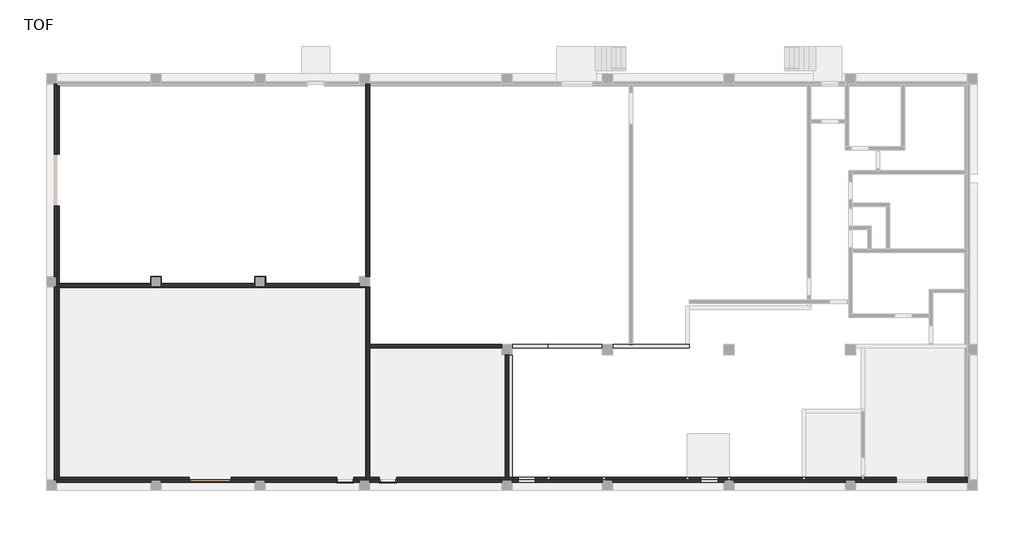
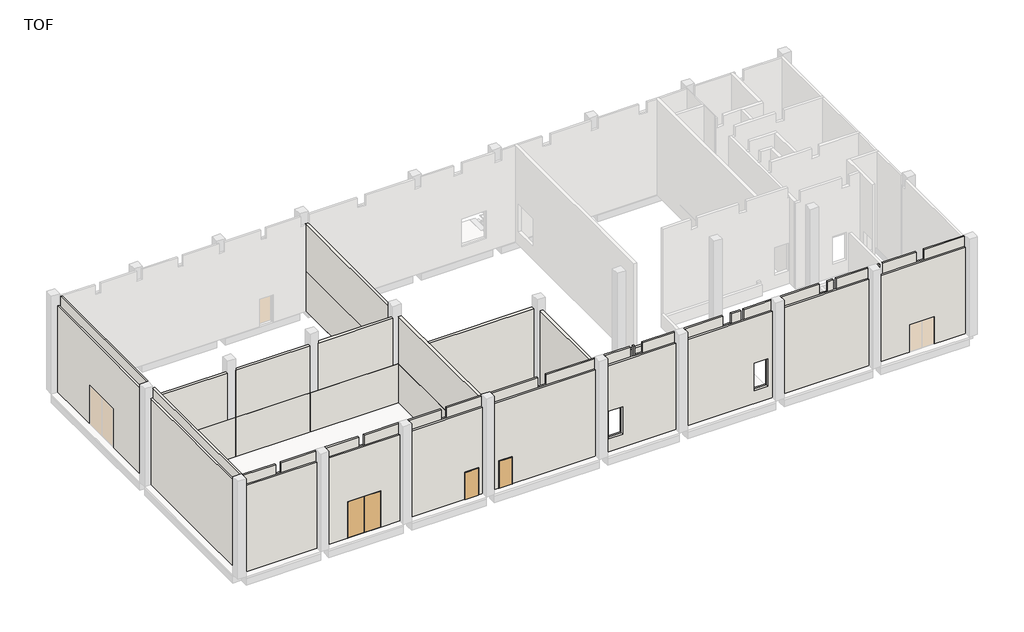
# One storey, part 1 of 4: 21 walls, 3 doors.
"""IFC4 building model written with IfcOpenShell, lengths in millimetres."""

import ifcopenshell
import ifcopenshell.guid

model = None  # the IFC model being written
_history = None  # IfcOwnerHistory: only IFC2X3 demands one
_inside = {}  # id of a spatial element -> (the spatial element, [elements in it])
_under = {}  # id of a project, library or spatial element -> (it, [spatial elements below it])
_declared = {}  # id of a project -> (the project, [libraries it declares])
_typed = {}  # id of a type object -> (the type object, [elements of that type])
_made_of = {}  # id of a material, layer set ... -> (it, [elements and type objects made of it])


def new_model(schema):
    """Start an empty IFC model of exactly this schema.

    Asked for "IFC4X3", IfcOpenShell would pick the latest addendum, in which some entities
    have other attributes; the version numbers below select the first issue.
    IFC2X3 requires an IfcOwnerHistory on every rooted entity: one is made here for all.
    """
    global model, _history
    if schema == "IFC4X3":
        model = ifcopenshell.file(schema_version=(4, 3, 0, 0))
    else:
        model = ifcopenshell.file(schema=schema)
    _inside.clear()
    _under.clear()
    _declared.clear()
    _typed.clear()
    _made_of.clear()
    _history = None
    if model.schema == "IFC2X3":
        org = make("IfcOrganization", Name="unknown")
        user = make(
            "IfcPersonAndOrganization",
            ThePerson=make("IfcPerson", FamilyName="unknown"),
            TheOrganization=org,
        )
        app = make(
            "IfcApplication",
            ApplicationDeveloper=org,
            Version="unknown",
            ApplicationFullName="unknown",
            ApplicationIdentifier="unknown",
        )
        _history = make(
            "IfcOwnerHistory",
            OwningUser=user,
            OwningApplication=app,
            ChangeAction="ADDED",
            CreationDate=0,
        )
    return model


def make(cls, **values):
    """One entity of the class cls with the attributes given. An attribute that is None is left unset."""
    return model.create_entity(
        cls, **{name: value for name, value in values.items() if value is not None}
    )


def rooted(cls, **values):
    """An entity with a GlobalId (a new one), such as an element, a storey or a relation."""
    return make(cls, GlobalId=ifcopenshell.guid.new(), OwnerHistory=_history, **values)


def si_unit(unit_type, name, prefix=None):
    """IfcSIUnit, for example si_unit("LENGTHUNIT", "METRE", prefix="MILLI")."""
    return make("IfcSIUnit", UnitType=unit_type, Prefix=prefix, Name=name)


def assignment(units):
    """IfcUnitAssignment: the units of a project."""
    return None if units is None else make("IfcUnitAssignment", Units=units)


def point(xyz):
    """IfcCartesianPoint."""
    return None if xyz is None else make("IfcCartesianPoint", Coordinates=xyz)


def direction(xyz):
    """IfcDirection."""
    return None if xyz is None else make("IfcDirection", DirectionRatios=xyz)


def frame(location, z_axis=None, x_axis=None):
    """IfcAxis2Placement3D, a coordinate frame: its origin and axes. An axis left out is left unset."""
    return make(
        "IfcAxis2Placement3D",
        Location=point(location),
        Axis=direction(z_axis),
        RefDirection=direction(x_axis),
    )


def origin():
    """The frame at (0, 0, 0) with its axes left unset."""
    return frame((0.0, 0.0, 0.0))


def origin_with_axes():
    """The frame at (0, 0, 0) with the z axis (0, 0, 1) and the x axis (1, 0, 0) written out."""
    return frame((0.0, 0.0, 0.0), z_axis=(0.0, 0.0, 1.0), x_axis=(1.0, 0.0, 0.0))


def place(relative_to, where):
    """IfcLocalPlacement: puts the frame where relative to a parent placement (None: the world)."""
    return make(
        "IfcLocalPlacement", PlacementRelTo=relative_to, RelativePlacement=where
    )


def context(
    kind, dimensions, precision=None, world=None, true_north=None, identifier=None
):
    """IfcGeometricRepresentationContext, for example the 3D "Model" context."""
    return make(
        "IfcGeometricRepresentationContext",
        ContextIdentifier=identifier,
        ContextType=kind,
        CoordinateSpaceDimension=dimensions,
        Precision=precision,
        WorldCoordinateSystem=world,
        TrueNorth=true_north,
    )


def project(units=None, contexts=None):
    """IfcProject with its units and contexts."""
    return rooted(
        "IfcProject",
        Name="project",
        RepresentationContexts=contexts,
        UnitsInContext=assignment(units),
    )


def spatial(cls, under=None, at=None, **own):
    """A site, building, storey or space (cls), placed at a placement, below another one or the project."""
    s = rooted(cls, ObjectPlacement=at, **own)
    if under is not None:
        _under.setdefault(under.id(), (under, []))[1].append(s)
    return s


def polyline(points):
    """IfcPolyline through the points."""
    return make("IfcPolyline", Points=[point(p) for p in points])


def outline(outer, holes=None, kind="AREA"):
    """IfcArbitraryClosedProfileDef: a profile drawn as a closed curve; with holes, ...WithVoids."""
    if holes is None:
        return make("IfcArbitraryClosedProfileDef", ProfileType=kind, OuterCurve=outer)
    return make(
        "IfcArbitraryProfileDefWithVoids",
        ProfileType=kind,
        OuterCurve=outer,
        InnerCurves=holes,
    )


def extrude(swept, where, along, depth):
    """IfcExtrudedAreaSolid: the profile swept, set in the frame where, extruded along a direction by depth."""
    return make(
        "IfcExtrudedAreaSolid",
        SweptArea=swept,
        Position=where,
        ExtrudedDirection=direction(along),
        Depth=depth,
    )


def faces_of(points, faces, orient=None, outer=None):
    """IfcFace entities. A face is a list of loops; a loop is a list of indices into points, from 0.

    orient and outer hold one flag for each loop. By default every Orientation is true, the
    first loop of a face is its IfcFaceOuterBound and the others are IfcFaceBound.
    """
    made = []
    for i, loops in enumerate(faces):
        bounds = []
        for j, loop in enumerate(loops):
            is_outer = j == 0 if outer is None else outer[i][j]
            bounds.append(
                make(
                    "IfcFaceOuterBound" if is_outer else "IfcFaceBound",
                    Bound=make("IfcPolyLoop", Polygon=[points[k] for k in loop]),
                    Orientation=True if orient is None else orient[i][j],
                )
            )
        made.append(make("IfcFace", Bounds=bounds))
    return made


def faceted_brep(points, faces, orient=None, outer=None, voids=None):
    """IfcFacetedBrep: a solid bounded by flat faces; with voids (closed shells), ...WithVoids."""
    shared = [point(p) for p in points]
    hull = make("IfcClosedShell", CfsFaces=faces_of(shared, faces, orient, outer))
    if voids is None:
        return make("IfcFacetedBrep", Outer=hull)
    return make(
        "IfcFacetedBrepWithVoids",
        Outer=hull,
        Voids=[
            make(cls, CfsFaces=faces_of(shared, fs, o, b)) for cls, fs, o, b in voids
        ],
    )


def shape(context_of_items, identifier, shape_type, items):
    """IfcShapeRepresentation: the items that make up one representation, for example the "Body"."""
    return make(
        "IfcShapeRepresentation",
        ContextOfItems=context_of_items,
        RepresentationIdentifier=identifier,
        RepresentationType=shape_type,
        Items=items,
    )


def source(mapping_origin, context_of_items, identifier, shape_type, items):
    """IfcRepresentationMap: a shape defined once, which mapped items show again and again."""
    return make(
        "IfcRepresentationMap",
        MappingOrigin=mapping_origin,
        MappedRepresentation=shape(context_of_items, identifier, shape_type, items),
    )


def transform(
    local_origin,
    x_axis=None,
    y_axis=None,
    z_axis=None,
    scale=None,
    scale2=None,
    scale3=None,
    uniform=True,
):
    """IfcCartesianTransformationOperator3D, or its non-uniform kind. x_axis, y_axis, z_axis: its Axis1, 2, 3."""
    if uniform:
        return make(
            "IfcCartesianTransformationOperator3D",
            Axis1=direction(x_axis),
            Axis2=direction(y_axis),
            LocalOrigin=point(local_origin),
            Scale=scale,
            Axis3=direction(z_axis),
        )
    return make(
        "IfcCartesianTransformationOperator3DnonUniform",
        Axis1=direction(x_axis),
        Axis2=direction(y_axis),
        LocalOrigin=point(local_origin),
        Scale=scale,
        Axis3=direction(z_axis),
        Scale2=scale2,
        Scale3=scale3,
    )


def mapped(mapping_source, mapping_target):
    """IfcMappedItem: shows the shape of a source again, moved by a transform."""
    return make(
        "IfcMappedItem", MappingSource=mapping_source, MappingTarget=mapping_target
    )


def made_of(thing, what):
    """Note that an element or type object is made of a material, layer set ...; save() writes the relation."""
    if what is not None:
        _made_of.setdefault(what.id(), (what, []))[1].append(thing)
    return thing


def element(
    cls,
    number,
    at=None,
    inside=None,
    cuts=None,
    type_object=None,
    material=None,
    context=None,
    identifier="Body",
    shape_type=None,
    held_by="IfcProductDefinitionShape",
    body=None,
    shapes=None,
    **own,
):
    """One element of the class cls, such as IfcWall. Its Tag is "e" and its number.

    at: its placement. inside: the storey or other place that contains it. cuts: it is an
    opening in that element (IfcRelVoidsElement). A single representation is given by context,
    identifier, shape_type and body (its items); several are given by shapes. held_by: the class
    of the entity that holds the representations. save() writes the other relations.
    """
    e = rooted(cls, Tag="e%d" % number, ObjectPlacement=at, **own)
    if body is not None:
        shapes = [shape(context, identifier, shape_type, body)]
    if shapes is not None:
        e.Representation = make(held_by, Representations=shapes)
    if inside is not None:
        _inside.setdefault(inside.id(), (inside, []))[1].append(e)
    if cuts is not None:
        rooted(
            "IfcRelVoidsElement", RelatingBuildingElement=cuts, RelatedOpeningElement=e
        )
    if type_object is not None:
        _typed.setdefault(type_object.id(), (type_object, []))[1].append(e)
    return made_of(e, material)


def aggregate(whole, parts):
    """IfcRelAggregates: a whole, such as a stair, and the parts it consists of."""
    return rooted("IfcRelAggregates", RelatingObject=whole, RelatedObjects=parts)


def save(model, path):
    """Write the relations noted so far, then the file.

    IfcRelAggregates (storeys below a building ...), IfcRelContainedInSpatialStructure (elements
    in a storey), IfcRelDefinesByType, IfcRelAssociatesMaterial and IfcRelDeclares: one each for
    every whole, place, type object, material and project.
    """
    for whole, parts in _under.values():
        aggregate(whole, parts)
    for where, things in _inside.values():
        rooted(
            "IfcRelContainedInSpatialStructure",
            RelatedElements=things,
            RelatingStructure=where,
        )
    for kind, things in _typed.values():
        rooted("IfcRelDefinesByType", RelatedObjects=things, RelatingType=kind)
    for what, things in _made_of.values():
        rooted("IfcRelAssociatesMaterial", RelatedObjects=things, RelatingMaterial=what)
    for by, libraries in _declared.values():
        rooted("IfcRelDeclares", RelatingContext=by, RelatedDefinitions=libraries)
    model.write(path)


def double_door_steel_3c62acbf(model_context):
    return source(origin(), model_context, "Body", "SolidModel", [
        extrude(outline(polyline([(1180.0, 35.0), (0.0, 35.0), (0.0, 75.0), (1180.0, 75.0), (1180.0, 35.0)])), frame((0.0, 0.0, 20.0), z_axis=(0.0, 0.0, 1.0), x_axis=(1.0, 0.0, 0.0)), (0.0, 0.0, 1.0), 2760.0),
        extrude(outline(polyline([(0.0, 35.0), (-1180.0, 35.0), (-1180.0, 75.0), (0.0, 75.0), (0.0, 35.0)])), frame((0.0, 0.0, 20.0), z_axis=(0.0, 0.0, 1.0), x_axis=(1.0, 0.0, 0.0)), (0.0, 0.0, 1.0), 2760.0),
        faceted_brep([(1200.0, -75.0, 2800.0), (1200.0, 75.0, 2800.0), (-1200.0, 75.0, 2800.0), (-1200.0, -75.0, 2800.0), (1165.0, 35.0, 2765.0), (1165.0, -75.0, 2765.0), (-1165.0, -75.0, 2765.0), (-1165.0, 35.0, 2765.0), (1180.0, 75.0, 2780.0), (1180.0, 35.0, 2780.0), (-1180.0, 35.0, 2780.0), (-1180.0, 75.0, 2780.0), (-1200.0, 75.0, 0.0), (-1200.0, -75.0, 0.0), (-1165.0, -75.0, 35.0), (-1165.0, 35.0, 35.0), (-1180.0, 35.0, 20.0), (-1180.0, 75.0, 20.0), (1200.0, 75.0, 0.0), (1180.0, 75.0, 20.0), (1200.0, -75.0, 0.0), (1165.0, -75.0, 35.0), (1165.0, 35.0, 35.0), (1180.0, 35.0, 20.0)], [[[0, 1, 2, 3]], [[4, 5, 6, 7]], [[8, 9, 10, 11]], [[3, 2, 12, 13]], [[7, 6, 14, 15]], [[11, 10, 16, 17]], [[18, 12, 2, 1], [8, 11, 17, 19]], [[13, 12, 18, 20]], [[0, 3, 13, 20], [21, 14, 6, 5]], [[15, 14, 21, 22]], [[23, 16, 10, 9], [4, 7, 15, 22]], [[17, 16, 23, 19]], [[20, 18, 1, 0]], [[22, 21, 5, 4]], [[19, 23, 9, 8]]]),
    ])


def single_door_steel_8d57826b(model_context):
    return source(origin(), model_context, "Body", "SolidModel", [
        extrude(outline(polyline([(470.0, -105.0), (-470.0, -105.0), (-470.0, -70.0), (470.0, -70.0), (470.0, -105.0)])), origin_with_axes(), (0.0, 0.0, 1.0), 2070.0),
        faceted_brep([(470.0, -105.0, 0.0), (470.0, -70.0, 0.0), (450.0, -70.0, 0.0), (450.0, 70.0, 0.0), (470.0, 70.0, 0.0), (470.0, 105.0, 0.0), (500.0, 105.0, 0.0), (500.0, -105.0, 0.0), (500.0, -105.0, 2100.0), (-500.0, -105.0, 2100.0), (-500.0, -105.0, 0.0), (-470.0, -105.0, 0.0), (-470.0, -105.0, 2070.0), (470.0, -105.0, 2070.0), (500.0, 105.0, 2100.0), (470.0, 105.0, 2070.0), (-470.0, 105.0, 2070.0), (-470.0, 105.0, 0.0), (-500.0, 105.0, 0.0), (-500.0, 105.0, 2100.0), (470.0, 70.0, 2070.0), (450.0, 70.0, 2050.0), (-450.0, 70.0, 2050.0), (-450.0, 70.0, 0.0), (-470.0, 70.0, 0.0), (-470.0, 70.0, 2070.0), (450.0, -70.0, 2050.0), (470.0, -70.0, 2070.0), (-470.0, -70.0, 2070.0), (-470.0, -70.0, 0.0), (-450.0, -70.0, 0.0), (-450.0, -70.0, 2050.0)], [[[0, 1, 2, 3, 4, 5, 6, 7]], [[7, 8, 9, 10, 11, 12, 13, 0]], [[6, 14, 8, 7]], [[5, 15, 16, 17, 18, 19, 14, 6]], [[4, 20, 15, 5]], [[3, 21, 22, 23, 24, 25, 20, 4]], [[2, 26, 21, 3]], [[1, 27, 28, 29, 30, 31, 26, 2]], [[0, 13, 27, 1]], [[12, 11, 29, 28]], [[11, 10, 18, 17, 24, 23, 30, 29]], [[19, 18, 10, 9]], [[25, 24, 17, 16]], [[31, 30, 23, 22]], [[14, 19, 9, 8]], [[20, 25, 16, 15]], [[26, 31, 22, 21]], [[13, 12, 28, 27]]]),
    ])


def single_door_steel_6218e75e(model_context):
    return source(origin(), model_context, "Body", "SolidModel", [
        extrude(outline(polyline([(470.0, 105.0), (470.0, 70.0), (-470.0, 70.0), (-470.0, 105.0), (470.0, 105.0)])), origin_with_axes(), (0.0, 0.0, 1.0), 2070.0),
        faceted_brep([(470.0, 105.0, 0.0), (500.0, 105.0, 0.0), (500.0, -105.0, 0.0), (470.0, -105.0, 0.0), (470.0, -70.0, 0.0), (450.0, -70.0, 0.0), (450.0, 70.0, 0.0), (470.0, 70.0, 0.0), (470.0, 105.0, 2070.0), (-470.0, 105.0, 2070.0), (-470.0, 105.0, 0.0), (-500.0, 105.0, 0.0), (-500.0, 105.0, 2100.0), (500.0, 105.0, 2100.0), (500.0, -105.0, 2100.0), (-500.0, -105.0, 2100.0), (-500.0, -105.0, 0.0), (-470.0, -105.0, 0.0), (-470.0, -105.0, 2070.0), (470.0, -105.0, 2070.0), (470.0, -70.0, 2070.0), (-470.0, -70.0, 2070.0), (-470.0, -70.0, 0.0), (-450.0, -70.0, 0.0), (-450.0, -70.0, 2050.0), (450.0, -70.0, 2050.0), (450.0, 70.0, 2050.0), (-450.0, 70.0, 2050.0), (-450.0, 70.0, 0.0), (-470.0, 70.0, 0.0), (-470.0, 70.0, 2070.0), (470.0, 70.0, 2070.0)], [[[0, 1, 2, 3, 4, 5, 6, 7]], [[1, 0, 8, 9, 10, 11, 12, 13]], [[2, 1, 13, 14]], [[3, 2, 14, 15, 16, 17, 18, 19]], [[4, 3, 19, 20]], [[5, 4, 20, 21, 22, 23, 24, 25]], [[6, 5, 25, 26]], [[7, 6, 26, 27, 28, 29, 30, 31]], [[0, 7, 31, 8]], [[9, 30, 29, 10]], [[10, 29, 28, 23, 22, 17, 16, 11]], [[15, 12, 11, 16]], [[21, 18, 17, 22]], [[27, 24, 23, 28]], [[14, 13, 12, 15]], [[20, 19, 18, 21]], [[26, 25, 24, 27]], [[8, 31, 30, 9]]]),
    ])


model = new_model("IFC4")

# Units and contexts
model_context = context("Model", 3, world=origin())
ifc_project = project(units=[si_unit("LENGTHUNIT", "METRE", prefix="MILLI")], contexts=[model_context])

# Site, building, storey
site = spatial("IfcSite", under=ifc_project)
building = spatial("IfcBuilding", under=site)
storey = spatial("IfcBuildingStorey", under=building, Name="TOF", Elevation=149.9618634)

# Doors
placement = place(None, origin())
double_door_steel_shape = double_door_steel_3c62acbf(model_context)
element("IfcDoor", 1, ObjectType="Double Door_Steel : H_DR_AR_B12_Double Door_Steel_W2400xH2800", at=placement, inside=storey, context=model_context, shape_type="MappedRepresentation", body=[
    mapped(double_door_steel_shape, transform((9125.0, 724.5208589, 149.9618634), x_axis=(-1.0, 0.0, 0.0), y_axis=(0.0, -1.0, 0.0), z_axis=(0.0, 0.0, 1.0))),
])
single_door_steel_shape = single_door_steel_8d57826b(model_context)
element("IfcDoor", 2, ObjectType="Single Door_Steel : H_DR_AR_B12_Single Door_Steel_W1000xH2100", at=placement, inside=storey, context=model_context, shape_type="MappedRepresentation", body=[
    mapped(single_door_steel_shape, transform((19350.0, 724.5208589, 149.9618634), x_axis=(1.0, 0.0, 0.0), y_axis=(0.0, 1.0, 0.0), z_axis=(0.0, 0.0, 1.0))),
])
single_door_steel_2_shape = single_door_steel_6218e75e(model_context)
element("IfcDoor", 3, ObjectType="Single Door_Steel : H_DR_AR_B12_Single Door_Steel_W1000xH2100", at=placement, inside=storey, context=model_context, shape_type="MappedRepresentation", body=[
    mapped(single_door_steel_2_shape, transform((16900.0, 724.5208589, 149.9618634), x_axis=(-1.0, 0.0, 0.0), y_axis=(0.0, -1.0, 0.0), z_axis=(0.0, 0.0, 1.0))),
])

# Walls
element("IfcWall", 4, ObjectType="H_WA_AR_B02_Ext Wall_RC T150", at=placement, inside=storey, context=model_context, shape_type="Brep", body=[
    faceted_brep([(300.0, 19574.5208589, 149.9618634), (300.0, 23473.5208589, 149.9618634), (300.0, 23599.5208589, 149.9618634), (300.0, 23599.5208589, 6749.9618634), (300.0, 12499.5208589, 6749.9618634), (300.0, 12499.5208589, 149.9618634), (300.0, 16574.5208589, 149.9618634), (300.0, 16574.5208589, 3149.9618634), (300.0, 19574.5208589, 3149.9618634), (150.0, 23599.5208589, 149.9618634), (150.0, 19574.5208589, 149.9618634), (150.0, 19574.5208589, 3149.9618634), (150.0, 16574.5208589, 3149.9618634), (150.0, 16574.5208589, 149.9618634), (150.0, 12499.5208589, 149.9618634), (150.0, 12499.5208589, 6749.9618634), (150.0, 23599.5208589, 6749.9618634)], [[[0, 1, 2, 3, 4, 5, 6, 7, 8]], [[9, 10, 11, 12, 13, 14, 15, 16]], [[13, 6, 5, 14]], [[2, 1, 0, 10, 9]], [[8, 11, 10, 0]], [[11, 8, 7, 12]], [[12, 7, 6, 13]], [[14, 5, 4, 15]], [[2, 9, 16, 3]], [[4, 3, 16, 15]]]),
    faceted_brep([(300.0, 799.5208589, 149.9618634), (300.0, 11899.5208589, 149.9618634), (300.0, 11899.5208589, 6749.9618634), (300.0, 799.5208589, 6749.9618634), (150.0, 11899.5208589, 149.9618634), (150.0, 799.5208589, 149.9618634), (150.0, 799.5208589, 6749.9618634), (150.0, 11899.5208589, 6749.9618634)], [[[0, 1, 2, 3]], [[4, 5, 6, 7]], [[4, 1, 0, 5]], [[1, 4, 7, 2]], [[5, 0, 3, 6]], [[7, 6, 3, 2]]]),
])
element("IfcWall", 5, ObjectType="H_WA_AR_B02_Ext Wall_RC T150", at=placement, inside=storey, context=model_context, shape_type="Brep", body=[
    faceted_brep([(7925.0, 799.5208589, 2949.9618634), (7925.0, 799.5208589, 149.9618634), (6300.0, 799.5208589, 149.9618634), (6300.0, 799.5208589, 6749.9618634), (8800.0, 799.5208589, 6749.9618634), (9200.0, 799.5208589, 6749.9618634), (11700.0, 799.5208589, 6749.9618634), (11700.0, 799.5208589, 149.9618634), (10325.0, 799.5208589, 149.9618634), (10325.0, 799.5208589, 2949.9618634), (7925.0, 649.5208589, 149.9618634), (7925.0, 649.5208589, 2949.9618634), (10325.0, 649.5208589, 2949.9618634), (10325.0, 649.5208589, 149.9618634), (11700.0, 649.5208589, 149.9618634), (11700.0, 649.5208589, 6749.9618634), (6300.0, 649.5208589, 6749.9618634), (6300.0, 649.5208589, 149.9618634)], [[[0, 1, 2, 3, 4, 5, 6, 7, 8, 9]], [[10, 11, 12, 13, 14, 15, 16, 17]], [[1, 10, 17, 2]], [[13, 8, 7, 14]], [[0, 11, 10, 1]], [[11, 0, 9, 12]], [[12, 9, 8, 13]], [[2, 17, 16, 3]], [[14, 7, 6, 15]], [[6, 5, 4, 3, 16, 15]]]),
    faceted_brep([(19850.0, 799.5208589, 149.9618634), (19850.0, 799.5208589, 2249.9618634), (18850.0, 799.5208589, 2249.9618634), (18850.0, 799.5208589, 149.9618634), (18300.0, 799.5208589, 149.9618634), (18300.0, 799.5208589, 6749.9618634), (21800.0, 799.5208589, 6749.9618634), (22400.0, 799.5208589, 6749.9618634), (25900.0, 799.5208589, 6749.9618634), (25900.0, 799.5208589, 149.9618634), (19850.0, 649.5208589, 2249.9618634), (19850.0, 649.5208589, 149.9618634), (25900.0, 649.5208589, 149.9618634), (25900.0, 649.5208589, 6749.9618634), (18300.0, 649.5208589, 6749.9618634), (18300.0, 649.5208589, 149.9618634), (18850.0, 649.5208589, 149.9618634), (18850.0, 649.5208589, 2249.9618634)], [[[0, 1, 2, 3, 4, 5, 6, 7, 8, 9]], [[10, 11, 12, 13, 14, 15, 16, 17]], [[11, 0, 9, 12]], [[3, 16, 15, 4]], [[10, 1, 0, 11]], [[1, 10, 17, 2]], [[2, 17, 16, 3]], [[4, 15, 14, 5]], [[12, 9, 8, 13]], [[8, 7, 6, 5, 14, 13]]]),
    faceted_brep([(16400.0, 799.5208589, 2249.9618634), (16400.0, 799.5208589, 149.9618634), (12300.0, 799.5208589, 149.9618634), (12300.0, 799.5208589, 6749.9618634), (14800.0, 799.5208589, 6749.9618634), (15200.0, 799.5208589, 6749.9618634), (17700.0, 799.5208589, 6749.9618634), (17700.0, 799.5208589, 149.9618634), (17400.0, 799.5208589, 149.9618634), (17400.0, 799.5208589, 2249.9618634), (16400.0, 649.5208589, 149.9618634), (16400.0, 649.5208589, 2249.9618634), (17400.0, 649.5208589, 2249.9618634), (17400.0, 649.5208589, 149.9618634), (17700.0, 649.5208589, 149.9618634), (17700.0, 649.5208589, 6749.9618634), (12300.0, 649.5208589, 6749.9618634), (12300.0, 649.5208589, 149.9618634)], [[[0, 1, 2, 3, 4, 5, 6, 7, 8, 9]], [[10, 11, 12, 13, 14, 15, 16, 17]], [[1, 10, 17, 2]], [[13, 8, 7, 14]], [[0, 11, 10, 1]], [[11, 0, 9, 12]], [[12, 9, 8, 13]], [[14, 7, 6, 15]], [[2, 17, 16, 3]], [[6, 5, 4, 3, 16, 15]]]),
    faceted_brep([(48625.0, 799.5208589, 2249.9618634), (48625.0, 799.5208589, 149.9618634), (46800.0, 799.5208589, 149.9618634), (46600.0, 799.5208589, 149.9618634), (46300.0, 799.5208589, 149.9618634), (46300.0, 799.5208589, 6749.9618634), (49200.0, 799.5208589, 6749.9618634), (49800.0, 799.5208589, 6749.9618634), (52700.0, 799.5208589, 6749.9618634), (52700.0, 799.5208589, 149.9618634), (50425.0, 799.5208589, 149.9618634), (50425.0, 799.5208589, 2249.9618634), (48625.0, 649.5208589, 149.9618634), (48625.0, 649.5208589, 2249.9618634), (50425.0, 649.5208589, 2249.9618634), (50425.0, 649.5208589, 149.9618634), (52700.0, 649.5208589, 149.9618634), (52700.0, 649.5208589, 6749.9618634), (46300.0, 649.5208589, 6749.9618634), (46300.0, 649.5208589, 149.9618634)], [[[0, 1, 2, 3, 4, 5, 6, 7, 8, 9, 10, 11]], [[12, 13, 14, 15, 16, 17, 18, 19]], [[1, 12, 19, 4, 3, 2]], [[15, 10, 9, 16]], [[0, 13, 12, 1]], [[13, 0, 11, 14]], [[14, 11, 10, 15]], [[16, 9, 8, 17]], [[4, 19, 18, 5]], [[8, 7, 6, 5, 18, 17]]]),
    faceted_brep([(5700.0, 799.5208589, 149.9618634), (426.0, 799.5208589, 149.9618634), (300.0, 799.5208589, 149.9618634), (300.0, 799.5208589, 6749.9618634), (2800.0, 799.5208589, 6749.9618634), (3200.0, 799.5208589, 6749.9618634), (5700.0, 799.5208589, 6749.9618634), (300.0, 649.5208589, 149.9618634), (5700.0, 649.5208589, 149.9618634), (5700.0, 649.5208589, 6749.9618634), (300.0, 649.5208589, 6749.9618634)], [[[0, 1, 2, 3, 4, 5, 6]], [[7, 8, 9, 10]], [[7, 2, 1, 0, 8]], [[2, 7, 10, 3]], [[8, 0, 6, 9]], [[6, 5, 4, 3, 10, 9]]]),
    faceted_brep([(45700.0, 799.5208589, 149.9618634), (43400.0, 799.5208589, 149.9618634), (43200.0, 799.5208589, 149.9618634), (39300.0, 799.5208589, 149.9618634), (39300.0, 799.5208589, 6749.9618634), (42200.0, 799.5208589, 6749.9618634), (42800.0, 799.5208589, 6749.9618634), (45700.0, 799.5208589, 6749.9618634), (39300.0, 649.5208589, 149.9618634), (45700.0, 649.5208589, 149.9618634), (45700.0, 649.5208589, 6749.9618634), (39300.0, 649.5208589, 6749.9618634)], [[[0, 1, 2, 3, 4, 5, 6, 7]], [[8, 9, 10, 11]], [[0, 9, 8, 3, 2, 1]], [[9, 0, 7, 10]], [[3, 8, 11, 4]], [[7, 6, 5, 4, 11, 10]]]),
    faceted_brep([(38700.0, 799.5208589, 149.9618634), (32300.0, 799.5208589, 149.9618634), (32300.0, 799.5208589, 6749.9618634), (35200.0, 799.5208589, 6749.9618634), (35800.0, 799.5208589, 6749.9618634), (38700.0, 799.5208589, 6749.9618634), (37375.0, 799.5208589, 3249.9618634), (37375.0, 799.5208589, 1149.9618634), (38375.0, 799.5208589, 1149.9618634), (38375.0, 799.5208589, 3249.9618634), (32300.0, 649.5208589, 149.9618634), (38700.0, 649.5208589, 149.9618634), (38700.0, 649.5208589, 6749.9618634), (32300.0, 649.5208589, 6749.9618634), (37375.0, 649.5208589, 1149.9618634), (37375.0, 649.5208589, 3249.9618634), (38375.0, 649.5208589, 3249.9618634), (38375.0, 649.5208589, 1149.9618634)], [[[0, 1, 2, 3, 4, 5], [6, 7, 8, 9]], [[10, 11, 12, 13], [14, 15, 16, 17]], [[0, 11, 10, 1]], [[15, 14, 7, 6]], [[16, 15, 6, 9]], [[17, 16, 9, 8]], [[14, 17, 8, 7]], [[11, 0, 5, 12]], [[1, 10, 13, 2]], [[5, 4, 3, 2, 13, 12]]]),
    faceted_brep([(31700.0, 799.5208589, 149.9618634), (26500.0, 799.5208589, 149.9618634), (26500.0, 799.5208589, 6749.9618634), (28800.0, 799.5208589, 6749.9618634), (29400.0, 799.5208589, 6749.9618634), (31700.0, 799.5208589, 6749.9618634), (31700.0, 799.5208589, 1149.9618634), (27850.0, 799.5208589, 1149.9618634), (27850.0, 799.5208589, 3249.9618634), (26850.0, 799.5208589, 3249.9618634), (26850.0, 799.5208589, 1149.9618634), (26500.0, 649.5208589, 149.9618634), (31700.0, 649.5208589, 149.9618634), (31700.0, 649.5208589, 6749.9618634), (26500.0, 649.5208589, 6749.9618634), (27850.0, 649.5208589, 3249.9618634), (27850.0, 649.5208589, 1149.9618634), (26850.0, 649.5208589, 1149.9618634), (26850.0, 649.5208589, 3249.9618634)], [[[0, 1, 2, 3, 4, 5, 6], [7, 8, 9, 10]], [[11, 12, 13, 14], [15, 16, 17, 18]], [[11, 1, 0, 12]], [[8, 7, 16, 15]], [[9, 8, 15, 18]], [[10, 9, 18, 17]], [[7, 10, 17, 16]], [[1, 11, 14, 2]], [[12, 0, 6, 5, 13]], [[5, 4, 3, 2, 14, 13]]]),
])
element("IfcWall", 6, ObjectType="H_WA_AR_B02_Int Wall_Block T200", at=placement, inside=storey, context=model_context, shape_type="Brep", body=[
    faceted_brep([(12300.0, 11899.5208589, 149.9618634), (17700.0, 11899.5208589, 149.9618634), (17700.0, 11899.5208589, 6749.9618634), (12300.0, 11899.5208589, 6749.9618634), (17700.0, 12099.5208589, 149.9618634), (12300.0, 12099.5208589, 149.9618634), (12300.0, 12099.5208589, 6749.9618634), (17700.0, 12099.5208589, 6749.9618634)], [[[0, 1, 2, 3]], [[4, 5, 6, 7]], [[4, 1, 0, 5]], [[1, 4, 7, 2]], [[5, 0, 3, 6]], [[3, 2, 7, 6]]]),
    faceted_brep([(6300.0, 11899.5208589, 149.9618634), (11700.0, 11899.5208589, 149.9618634), (11700.0, 11899.5208589, 6749.9618634), (6300.0, 11899.5208589, 6749.9618634), (11700.0, 12099.5208589, 149.9618634), (6300.0, 12099.5208589, 149.9618634), (6300.0, 12099.5208589, 6749.9618634), (11700.0, 12099.5208589, 6749.9618634)], [[[0, 1, 2, 3]], [[4, 5, 6, 7]], [[4, 1, 0, 5]], [[1, 4, 7, 2]], [[5, 0, 3, 6]], [[3, 2, 7, 6]]]),
    faceted_brep([(300.0, 11899.5208589, 149.9618634), (426.0, 11899.5208589, 149.9618634), (5700.0, 11899.5208589, 149.9618634), (5700.0, 11899.5208589, 6749.9618634), (300.0, 11899.5208589, 6749.9618634), (5700.0, 12099.5208589, 149.9618634), (426.0, 12099.5208589, 149.9618634), (300.0, 12099.5208589, 149.9618634), (300.0, 12099.5208589, 6749.9618634), (426.0, 12099.5208589, 6749.9618634), (5700.0, 12099.5208589, 6749.9618634)], [[[0, 1, 2, 3, 4]], [[5, 6, 7, 8, 9, 10]], [[0, 7, 6, 5, 2, 1]], [[7, 0, 4, 8]], [[2, 5, 10, 3]], [[4, 3, 10, 9, 8]]]),
])
element("IfcWall", 7, ObjectType="H_WA_AR_B02_Int Wall_Block T200", at=placement, inside=storey, context=model_context, shape_type="Brep", body=[
    faceted_brep([(18100.0, 11899.5208589, 149.9618634), (18100.0, 925.5208589, 149.9618634), (18100.0, 799.5208589, 149.9618634), (18100.0, 799.5208589, 6749.9618634), (18100.0, 925.5208589, 6749.9618634), (18100.0, 11899.5208589, 6749.9618634), (18300.0, 799.5208589, 149.9618634), (18300.0, 925.5208589, 149.9618634), (18300.0, 8399.5208589, 149.9618634), (18300.0, 8599.5208589, 149.9618634), (18300.0, 11899.5208589, 149.9618634), (18300.0, 11899.5208589, 6749.9618634), (18300.0, 799.5208589, 6749.9618634)], [[[0, 1, 2, 3, 4, 5]], [[6, 7, 8, 9, 10, 11, 12]], [[6, 2, 1, 0, 10, 9, 8, 7]], [[2, 6, 12, 3]], [[10, 0, 5, 11]], [[5, 4, 3, 12, 11]]]),
    faceted_brep([(18100.0, 23599.5208589, 149.9618634), (18100.0, 23473.5208589, 149.9618634), (18100.0, 12499.5208589, 149.9618634), (18100.0, 12499.5208589, 6749.9618634), (18100.0, 23473.5208589, 6749.9618634), (18100.0, 23599.5208589, 6749.9618634), (18300.0, 12499.5208589, 149.9618634), (18300.0, 23473.5208589, 149.9618634), (18300.0, 23599.5208589, 149.9618634), (18300.0, 23599.5208589, 6749.9618634), (18300.0, 12499.5208589, 6749.9618634)], [[[0, 1, 2, 3, 4, 5]], [[6, 7, 8, 9, 10]], [[0, 8, 7, 6, 2, 1]], [[8, 0, 5, 9]], [[2, 6, 10, 3]], [[5, 4, 3, 10, 9]]]),
])
element("IfcWall", 8, ObjectType="H_WA_AR_B02_Int Wall_Block T200", at=placement, inside=storey, context=model_context, shape_type="Brep", body=[
    faceted_brep([(26100.0, 7999.5208589, 149.9618634), (26100.0, 925.5208589, 149.9618634), (26100.0, 799.5208589, 149.9618634), (26100.0, 799.5208589, 6749.9618634), (26100.0, 925.5208589, 6749.9618634), (26100.0, 7999.5208589, 6749.9618634), (26100.0, 7999.5208589, 1149.9618634), (26100.0, 2737.0208589, 1149.9618634), (26100.0, 2737.0208589, 999.9618634), (26100.0, 7999.5208589, 999.9618634), (26300.0, 799.5208589, 149.9618634), (26300.0, 925.5208589, 149.9618634), (26300.0, 7999.5208589, 149.9618634), (26300.0, 7999.5208589, 999.9618634), (26300.0, 2737.0208589, 999.9618634), (26300.0, 2737.0208589, 1149.9618634), (26300.0, 2837.0208589, 1149.9618634), (26300.0, 7999.5208589, 1149.9618634), (26300.0, 7999.5208589, 6749.9618634), (26300.0, 2837.0208589, 6749.9618634), (26300.0, 2637.0208589, 6749.9618634), (26300.0, 925.5208589, 6749.9618634), (26300.0, 799.5208589, 6749.9618634)], [[[0, 1, 2, 3, 4, 5, 6, 7, 8, 9]], [[10, 11, 12, 13, 14, 15, 16, 17, 18, 19, 20, 21, 22]], [[10, 2, 1, 0, 12, 11]], [[2, 10, 22, 3]], [[12, 0, 9, 13]], [[5, 18, 17, 6]], [[5, 4, 3, 22, 21, 20, 19, 18]], [[8, 14, 13, 9]], [[15, 7, 6, 17, 16]], [[14, 8, 7, 15]]]),
])
element("IfcWall", 9, ObjectType="H_WA_AR_B07_Int Wall_Plaster T12", at=placement, inside=storey, context=model_context, shape_type="Brep", body=[
    faceted_brep([(6300.0, 12511.5208589, 149.9618634), (6300.0, 12499.5208589, 149.9618634), (6300.0, 12099.5208589, 149.9618634), (6300.0, 12099.5208589, 3149.9618634), (6300.0, 12499.5208589, 3149.9618634), (6300.0, 12511.5208589, 3149.9618634), (6312.0, 12511.5208589, 149.9618634), (6312.0, 12511.5208589, 3149.9618634), (6312.0, 12111.5208589, 3149.9618634), (6312.0, 12099.5208589, 3149.9618634), (6312.0, 12099.5208589, 149.9618634), (6312.0, 12111.5208589, 149.9618634)], [[[0, 1, 2, 3, 4, 5]], [[6, 7, 8, 9, 10, 11]], [[2, 1, 0, 6, 11, 10]], [[5, 4, 3, 9, 8, 7]], [[0, 5, 7, 6]], [[3, 2, 10, 9]]]),
])
element("IfcWall", 10, ObjectType="H_WA_AR_B07_Int Wall_Plaster T12", at=placement, inside=storey, context=model_context, shape_type="Brep", body=[
    faceted_brep([(6312.0, 12099.5208589, 149.9618634), (11700.0, 12099.5208589, 149.9618634), (11700.0, 12099.5208589, 3149.9618634), (6312.0, 12099.5208589, 3149.9618634), (6312.0, 12111.5208589, 149.9618634), (6312.0, 12111.5208589, 3149.9618634), (11688.0, 12111.5208589, 3149.9618634), (11700.0, 12111.5208589, 3149.9618634), (11700.0, 12111.5208589, 149.9618634), (11688.0, 12111.5208589, 149.9618634)], [[[0, 1, 2, 3]], [[4, 5, 6, 7, 8, 9]], [[1, 0, 4, 9, 8]], [[3, 2, 7, 6, 5]], [[2, 1, 8, 7]], [[0, 3, 5, 4]]]),
])
element("IfcWall", 11, ObjectType="H_WA_AR_B07_Int Wall_Plaster T12", at=placement, inside=storey, context=model_context, shape_type="Brep", body=[
    faceted_brep([(11700.0, 12111.5208589, 149.9618634), (11700.0, 12499.5208589, 149.9618634), (11700.0, 12511.5208589, 149.9618634), (11700.0, 12511.5208589, 3149.9618634), (11700.0, 12499.5208589, 3149.9618634), (11700.0, 12111.5208589, 3149.9618634), (11688.0, 12111.5208589, 149.9618634), (11688.0, 12111.5208589, 3149.9618634), (11688.0, 12511.5208589, 3149.9618634), (11688.0, 12511.5208589, 149.9618634)], [[[0, 1, 2, 3, 4, 5]], [[6, 7, 8, 9]], [[2, 1, 0, 6, 9]], [[5, 4, 3, 8, 7]], [[3, 2, 9, 8]], [[0, 5, 7, 6]]]),
])
element("IfcWall", 12, ObjectType="H_WA_AR_B07_Int Wall_Plaster T12", at=placement, inside=storey, context=model_context, shape_type="Brep", body=[
    faceted_brep([(11700.0, 12499.5208589, 149.9618634), (12300.0, 12499.5208589, 149.9618634), (12312.0, 12499.5208589, 149.9618634), (12312.0, 12499.5208589, 3149.9618634), (12300.0, 12499.5208589, 3149.9618634), (11700.0, 12499.5208589, 3149.9618634), (11700.0, 12511.5208589, 149.9618634), (11700.0, 12511.5208589, 3149.9618634), (12312.0, 12511.5208589, 3149.9618634), (12312.0, 12511.5208589, 149.9618634)], [[[0, 1, 2, 3, 4, 5]], [[6, 7, 8, 9]], [[2, 1, 0, 6, 9]], [[5, 4, 3, 8, 7]], [[3, 2, 9, 8]], [[0, 5, 7, 6]]]),
])
element("IfcWall", 13, ObjectType="H_WA_AR_B07_Int Wall_Plaster T12", at=placement, inside=storey, context=model_context, shape_type="Brep", body=[
    faceted_brep([(12300.0, 12499.5208589, 149.9618634), (12300.0, 12099.5208589, 149.9618634), (12300.0, 12099.5208589, 3149.9618634), (12300.0, 12499.5208589, 3149.9618634), (12312.0, 12499.5208589, 149.9618634), (12312.0, 12499.5208589, 3149.9618634), (12312.0, 12111.5208589, 3149.9618634), (12312.0, 12099.5208589, 3149.9618634), (12312.0, 12099.5208589, 149.9618634), (12312.0, 12111.5208589, 149.9618634)], [[[0, 1, 2, 3]], [[4, 5, 6, 7, 8, 9]], [[1, 0, 4, 9, 8]], [[3, 2, 7, 6, 5]], [[2, 1, 8, 7]], [[0, 3, 5, 4]]]),
])
element("IfcWall", 14, ObjectType="H_WA_AR_B07_Int Wall_Plaster T12", at=placement, inside=storey, context=model_context, shape_type="SweptSolid", body=[
    extrude(outline(polyline([(17694.0, 12099.5208589), (12312.0, 12099.5208589), (12312.0, 12111.5208589), (17694.0, 12111.5208589), (17694.0, 12099.5208589)])), frame((0.0, 0.0, 149.9618634), z_axis=(0.0, 0.0, 1.0), x_axis=(1.0, 0.0, 0.0)), (0.0, 0.0, 1.0), 3000.0),
])
element("IfcWall", 15, ObjectType="H_WA_AR_B07_Int Wall_Plaster T12", at=placement, inside=storey, context=model_context, shape_type="Brep", body=[
    faceted_brep([(426.0, 12099.5208589, 149.9618634), (5700.0, 12099.5208589, 149.9618634), (5700.0, 12099.5208589, 3149.9618634), (426.0, 12099.5208589, 3149.9618634), (426.0, 12111.5208589, 149.9618634), (426.0, 12111.5208589, 3149.9618634), (5688.0, 12111.5208589, 3149.9618634), (5700.0, 12111.5208589, 3149.9618634), (5700.0, 12111.5208589, 149.9618634), (5688.0, 12111.5208589, 149.9618634)], [[[0, 1, 2, 3]], [[4, 5, 6, 7, 8, 9]], [[1, 0, 4, 9, 8]], [[3, 2, 7, 6, 5]], [[0, 3, 5, 4]], [[2, 1, 8, 7]]]),
])
element("IfcWall", 16, ObjectType="H_WA_AR_B07_Int Wall_Plaster T12", at=placement, inside=storey, context=model_context, shape_type="Brep", body=[
    faceted_brep([(5700.0, 12111.5208589, 149.9618634), (5700.0, 12499.5208589, 149.9618634), (5700.0, 12511.5208589, 149.9618634), (5700.0, 12511.5208589, 3149.9618634), (5700.0, 12499.5208589, 3149.9618634), (5700.0, 12111.5208589, 3149.9618634), (5688.0, 12111.5208589, 149.9618634), (5688.0, 12111.5208589, 3149.9618634), (5688.0, 12511.5208589, 3149.9618634), (5688.0, 12511.5208589, 149.9618634)], [[[0, 1, 2, 3, 4, 5]], [[6, 7, 8, 9]], [[2, 1, 0, 6, 9]], [[5, 4, 3, 8, 7]], [[3, 2, 9, 8]], [[0, 5, 7, 6]]]),
])
element("IfcWall", 17, ObjectType="H_WA_AR_B07_Int Wall_Plaster T12", at=placement, inside=storey, context=model_context, shape_type="SweptSolid", body=[
    extrude(outline(polyline([(6300.0, 12499.5208589), (5700.0, 12499.5208589), (5700.0, 12511.5208589), (6300.0, 12511.5208589), (6300.0, 12499.5208589)])), frame((0.0, 0.0, 149.9618634), z_axis=(0.0, 0.0, 1.0), x_axis=(1.0, 0.0, 0.0)), (0.0, 0.0, 1.0), 3000.0),
])
element("IfcWall", 18, ObjectType="H_WA_AR_B02_Ext Wall_1L Gypsum_Mineral Wool_T110", at=placement, inside=storey, context=model_context, shape_type="Brep", body=[
    faceted_brep([(426.0, 19574.5208589, 3149.9618634), (426.0, 19574.5208589, 149.9618634), (426.0, 23473.5208589, 149.9618634), (426.0, 23473.5208589, 7499.9618634), (426.0, 12499.5208589, 7499.9618634), (426.0, 12499.5208589, 6749.9618634), (426.0, 12099.5208589, 6749.9618634), (426.0, 12099.5208589, 149.9618634), (426.0, 16574.5208589, 149.9618634), (426.0, 16574.5208589, 3149.9618634), (300.0, 19574.5208589, 149.9618634), (300.0, 19574.5208589, 3149.9618634), (300.0, 16574.5208589, 3149.9618634), (300.0, 16574.5208589, 149.9618634), (300.0, 12499.5208589, 149.9618634), (300.0, 12099.5208589, 149.9618634), (300.0, 12099.5208589, 6749.9618634), (300.0, 12499.5208589, 6749.9618634), (300.0, 12499.5208589, 7499.9618634), (300.0, 23473.5208589, 7499.9618634), (300.0, 23473.5208589, 149.9618634)], [[[0, 1, 2, 3, 4, 5, 6, 7, 8, 9]], [[10, 11, 12, 13, 14, 15, 16, 17, 18, 19, 20]], [[1, 10, 20, 2]], [[13, 8, 7, 15, 14]], [[0, 11, 10, 1]], [[11, 0, 9, 12]], [[12, 9, 8, 13]], [[15, 7, 6, 16]], [[2, 20, 19, 3]], [[5, 17, 16, 6]], [[17, 5, 4, 18]], [[4, 3, 19, 18]]]),
    faceted_brep([(426.0, 799.5208589, 149.9618634), (426.0, 925.5208589, 149.9618634), (426.0, 11899.5208589, 149.9618634), (426.0, 11899.5208589, 6749.9618634), (426.0, 11899.5208589, 7499.9618634), (426.0, 925.5208589, 7499.9618634), (426.0, 799.5208589, 7499.9618634), (300.0, 11899.5208589, 149.9618634), (300.0, 799.5208589, 149.9618634), (300.0, 799.5208589, 6749.9618634), (300.0, 799.5208589, 7499.9618634), (300.0, 11899.5208589, 7499.9618634), (300.0, 11899.5208589, 6749.9618634)], [[[0, 1, 2, 3, 4, 5, 6]], [[7, 8, 9, 10, 11, 12]], [[0, 8, 7, 2, 1]], [[8, 0, 6, 10, 9]], [[2, 7, 12, 11, 4, 3]], [[6, 5, 4, 11, 10]]]),
])
element("IfcWall", 19, ObjectType="H_WA_AR_B02_Ext Wall_1L Gypsum_Mineral Wool_T110", at=placement, inside=storey, context=model_context, shape_type="Brep", body=[
    faceted_brep([(28500.0, 925.5208589, 1149.9618634), (28700.0, 925.5208589, 1149.9618634), (28700.0, 925.5208589, 7499.9618634), (28800.0, 925.5208589, 7499.9618634), (28800.0, 925.5208589, 6749.9618634), (29400.0, 925.5208589, 6749.9618634), (29400.0, 925.5208589, 7499.9618634), (31700.0, 925.5208589, 7499.9618634), (31700.0, 925.5208589, 1149.9618634), (31900.0, 925.5208589, 1149.9618634), (31900.0, 925.5208589, 6749.9618634), (32250.0, 925.5208589, 6749.9618634), (32250.0, 925.5208589, 7499.9618634), (35200.0, 925.5208589, 7499.9618634), (35200.0, 925.5208589, 6749.9618634), (35800.0, 925.5208589, 6749.9618634), (35800.0, 925.5208589, 7499.9618634), (36500.0, 925.5208589, 7499.9618634), (36500.0, 925.5208589, 1149.9618634), (36700.0, 925.5208589, 1149.9618634), (36700.0, 925.5208589, 7499.9618634), (38750.0, 925.5208589, 7499.9618634), (38750.0, 925.5208589, 6749.9618634), (38900.0, 925.5208589, 6749.9618634), (38900.0, 925.5208589, 1149.9618634), (39100.0, 925.5208589, 1149.9618634), (39100.0, 925.5208589, 6749.9618634), (39250.0, 925.5208589, 6749.9618634), (39250.0, 925.5208589, 7499.9618634), (42200.0, 925.5208589, 7499.9618634), (42200.0, 925.5208589, 6749.9618634), (42800.0, 925.5208589, 6749.9618634), (42800.0, 925.5208589, 7499.9618634), (43200.0, 925.5208589, 7499.9618634), (43200.0, 925.5208589, 1149.9618634), (43400.0, 925.5208589, 1149.9618634), (43400.0, 925.5208589, 7499.9618634), (45750.0, 925.5208589, 7499.9618634), (45750.0, 925.5208589, 6749.9618634), (46250.0, 925.5208589, 6749.9618634), (46250.0, 925.5208589, 7499.9618634), (46600.0, 925.5208589, 7499.9618634), (46600.0, 925.5208589, 149.9618634), (26500.0, 925.5208589, 149.9618634), (26300.0, 925.5208589, 149.9618634), (26300.0, 925.5208589, 1149.9618634), (26300.0, 925.5208589, 6749.9618634), (26450.0, 925.5208589, 6749.9618634), (26450.0, 925.5208589, 7499.9618634), (28500.0, 925.5208589, 7499.9618634), (27850.0, 925.5208589, 1149.9618634), (27850.0, 925.5208589, 3249.9618634), (26850.0, 925.5208589, 3249.9618634), (26850.0, 925.5208589, 1149.9618634), (37375.0, 925.5208589, 3249.9618634), (37375.0, 925.5208589, 1149.9618634), (38375.0, 925.5208589, 1149.9618634), (38375.0, 925.5208589, 3249.9618634), (28700.0, 799.5208589, 1149.9618634), (28500.0, 799.5208589, 1149.9618634), (28500.0, 799.5208589, 7499.9618634), (26500.0, 799.5208589, 7499.9618634), (26450.0, 799.5208589, 7499.9618634), (26450.0, 799.5208589, 6749.9618634), (26300.0, 799.5208589, 6749.9618634), (26300.0, 799.5208589, 149.9618634), (26500.0, 799.5208589, 149.9618634), (31700.0, 799.5208589, 149.9618634), (32300.0, 799.5208589, 149.9618634), (38700.0, 799.5208589, 149.9618634), (39300.0, 799.5208589, 149.9618634), (45700.0, 799.5208589, 149.9618634), (46300.0, 799.5208589, 149.9618634), (46600.0, 799.5208589, 149.9618634), (46600.0, 799.5208589, 7499.9618634), (46300.0, 799.5208589, 7499.9618634), (46250.0, 799.5208589, 7499.9618634), (46250.0, 799.5208589, 6749.9618634), (45750.0, 799.5208589, 6749.9618634), (45750.0, 799.5208589, 7499.9618634), (45700.0, 799.5208589, 7499.9618634), (43400.0, 799.5208589, 7499.9618634), (43400.0, 799.5208589, 1149.9618634), (43200.0, 799.5208589, 1149.9618634), (43200.0, 799.5208589, 7499.9618634), (42800.0, 799.5208589, 7499.9618634), (42800.0, 799.5208589, 6749.9618634), (42200.0, 799.5208589, 6749.9618634), (42200.0, 799.5208589, 7499.9618634), (39300.0, 799.5208589, 7499.9618634), (39250.0, 799.5208589, 7499.9618634), (39250.0, 799.5208589, 6749.9618634), (39100.0, 799.5208589, 6749.9618634), (39100.0, 799.5208589, 1149.9618634), (38900.0, 799.5208589, 1149.9618634), (38900.0, 799.5208589, 6749.9618634), (38750.0, 799.5208589, 6749.9618634), (38750.0, 799.5208589, 7499.9618634), (38700.0, 799.5208589, 7499.9618634), (36700.0, 799.5208589, 7499.9618634), (36700.0, 799.5208589, 1149.9618634), (36500.0, 799.5208589, 1149.9618634), (36500.0, 799.5208589, 7499.9618634), (35800.0, 799.5208589, 7499.9618634), (35800.0, 799.5208589, 6749.9618634), (35200.0, 799.5208589, 6749.9618634), (35200.0, 799.5208589, 7499.9618634), (32300.0, 799.5208589, 7499.9618634), (32250.0, 799.5208589, 7499.9618634), (32250.0, 799.5208589, 6749.9618634), (31900.0, 799.5208589, 6749.9618634), (31900.0, 799.5208589, 1149.9618634), (31700.0, 799.5208589, 1149.9618634), (31700.0, 799.5208589, 6749.9618634), (31700.0, 799.5208589, 7499.9618634), (29400.0, 799.5208589, 7499.9618634), (29400.0, 799.5208589, 6749.9618634), (28800.0, 799.5208589, 6749.9618634), (28800.0, 799.5208589, 7499.9618634), (28700.0, 799.5208589, 7499.9618634), (27850.0, 799.5208589, 3249.9618634), (27850.0, 799.5208589, 1149.9618634), (26850.0, 799.5208589, 1149.9618634), (26850.0, 799.5208589, 3249.9618634), (37375.0, 799.5208589, 1149.9618634), (37375.0, 799.5208589, 3249.9618634), (38375.0, 799.5208589, 3249.9618634), (38375.0, 799.5208589, 1149.9618634)], [[[0, 1, 2, 3, 4, 5, 6, 7, 8, 9, 10, 11, 12, 13, 14, 15, 16, 17, 18, 19, 20, 21, 22, 23, 24, 25, 26, 27, 28, 29, 30, 31, 32, 33, 34, 35, 36, 37, 38, 39, 40, 41, 42, 43, 44, 45, 46, 47, 48, 49], [50, 51, 52, 53], [54, 55, 56, 57]], [[58, 59, 60, 61, 62, 63, 64, 65, 66, 67, 68, 69, 70, 71, 72, 73, 74, 75, 76, 77, 78, 79, 80, 81, 82, 83, 84, 85, 86, 87, 88, 89, 90, 91, 92, 93, 94, 95, 96, 97, 98, 99, 100, 101, 102, 103, 104, 105, 106, 107, 108, 109, 110, 111, 112, 113, 114, 115, 116, 117, 118, 119], [120, 121, 122, 123], [124, 125, 126, 127]], [[65, 44, 43, 42, 73, 72, 71, 70, 69, 68, 67, 66]], [[44, 65, 64, 46, 45]], [[59, 0, 49, 60]], [[1, 58, 119, 2]], [[0, 59, 58, 1]], [[112, 8, 7, 114, 113]], [[9, 111, 110, 10]], [[8, 112, 111, 9]], [[101, 18, 17, 102]], [[19, 100, 99, 20]], [[18, 101, 100, 19]], [[25, 93, 92, 26]], [[94, 24, 23, 95]], [[93, 25, 24, 94]], [[35, 82, 81, 36]], [[83, 34, 33, 84]], [[82, 35, 34, 83]], [[73, 42, 41, 74]], [[51, 50, 121, 120]], [[52, 51, 120, 123]], [[53, 52, 123, 122]], [[50, 53, 122, 121]], [[125, 124, 55, 54]], [[126, 125, 54, 57]], [[127, 126, 57, 56]], [[124, 127, 56, 55]], [[47, 63, 62, 48]], [[63, 47, 46, 64]], [[11, 109, 108, 12]], [[109, 11, 10, 110]], [[27, 91, 90, 28]], [[91, 27, 26, 92]], [[22, 96, 95, 23]], [[96, 22, 21, 97]], [[39, 77, 76, 40]], [[77, 39, 38, 78]], [[78, 38, 37, 79]], [[117, 4, 3, 118]], [[4, 117, 116, 5]], [[5, 116, 115, 6]], [[105, 14, 13, 106]], [[14, 105, 104, 15]], [[15, 104, 103, 16]], [[87, 30, 29, 88]], [[30, 87, 86, 31]], [[31, 86, 85, 32]], [[49, 48, 62, 61, 60]], [[3, 2, 119, 118]], [[7, 6, 115, 114]], [[13, 12, 108, 107, 106]], [[17, 16, 103, 102]], [[21, 20, 99, 98, 97]], [[29, 28, 90, 89, 88]], [[33, 32, 85, 84]], [[37, 36, 81, 80, 79]], [[41, 40, 76, 75, 74]]]),
    faceted_brep([(18100.0, 925.5208589, 6749.9618634), (18100.0, 925.5208589, 149.9618634), (17400.0, 925.5208589, 149.9618634), (17400.0, 925.5208589, 2249.9618634), (16400.0, 925.5208589, 2249.9618634), (16400.0, 925.5208589, 149.9618634), (10325.0, 925.5208589, 149.9618634), (10325.0, 925.5208589, 2949.9618634), (7925.0, 925.5208589, 2949.9618634), (7925.0, 925.5208589, 149.9618634), (426.0, 925.5208589, 149.9618634), (426.0, 925.5208589, 7499.9618634), (2800.0, 925.5208589, 7499.9618634), (2800.0, 925.5208589, 6749.9618634), (3200.0, 925.5208589, 6749.9618634), (3200.0, 925.5208589, 7499.9618634), (5800.0, 925.5208589, 7499.9618634), (5800.0, 925.5208589, 6749.9618634), (6200.0, 925.5208589, 6749.9618634), (6200.0, 925.5208589, 7499.9618634), (8800.0, 925.5208589, 7499.9618634), (8800.0, 925.5208589, 6749.9618634), (9200.0, 925.5208589, 6749.9618634), (9200.0, 925.5208589, 7499.9618634), (11800.0, 925.5208589, 7499.9618634), (11800.0, 925.5208589, 6749.9618634), (12200.0, 925.5208589, 6749.9618634), (12200.0, 925.5208589, 7499.9618634), (14800.0, 925.5208589, 7499.9618634), (14800.0, 925.5208589, 6749.9618634), (15200.0, 925.5208589, 6749.9618634), (15200.0, 925.5208589, 7499.9618634), (17700.0, 925.5208589, 7499.9618634), (17700.0, 925.5208589, 6749.9618634), (18100.0, 799.5208589, 149.9618634), (18100.0, 799.5208589, 6749.9618634), (17700.0, 799.5208589, 6749.9618634), (17700.0, 799.5208589, 7499.9618634), (15200.0, 799.5208589, 7499.9618634), (15200.0, 799.5208589, 6749.9618634), (14800.0, 799.5208589, 6749.9618634), (14800.0, 799.5208589, 7499.9618634), (12300.0, 799.5208589, 7499.9618634), (12200.0, 799.5208589, 7499.9618634), (12200.0, 799.5208589, 6749.9618634), (11800.0, 799.5208589, 6749.9618634), (11800.0, 799.5208589, 7499.9618634), (11700.0, 799.5208589, 7499.9618634), (9200.0, 799.5208589, 7499.9618634), (9200.0, 799.5208589, 6749.9618634), (8800.0, 799.5208589, 6749.9618634), (8800.0, 799.5208589, 7499.9618634), (6300.0, 799.5208589, 7499.9618634), (6200.0, 799.5208589, 7499.9618634), (6200.0, 799.5208589, 6749.9618634), (5800.0, 799.5208589, 6749.9618634), (5800.0, 799.5208589, 7499.9618634), (5700.0, 799.5208589, 7499.9618634), (3200.0, 799.5208589, 7499.9618634), (3200.0, 799.5208589, 6749.9618634), (2800.0, 799.5208589, 6749.9618634), (2800.0, 799.5208589, 7499.9618634), (426.0, 799.5208589, 7499.9618634), (426.0, 799.5208589, 149.9618634), (5700.0, 799.5208589, 149.9618634), (6300.0, 799.5208589, 149.9618634), (7925.0, 799.5208589, 149.9618634), (7925.0, 799.5208589, 2949.9618634), (10325.0, 799.5208589, 2949.9618634), (10325.0, 799.5208589, 149.9618634), (11700.0, 799.5208589, 149.9618634), (12300.0, 799.5208589, 149.9618634), (16400.0, 799.5208589, 149.9618634), (16400.0, 799.5208589, 2249.9618634), (17400.0, 799.5208589, 2249.9618634), (17400.0, 799.5208589, 149.9618634), (17700.0, 799.5208589, 149.9618634)], [[[0, 1, 2, 3, 4, 5, 6, 7, 8, 9, 10, 11, 12, 13, 14, 15, 16, 17, 18, 19, 20, 21, 22, 23, 24, 25, 26, 27, 28, 29, 30, 31, 32, 33]], [[34, 35, 36, 37, 38, 39, 40, 41, 42, 43, 44, 45, 46, 47, 48, 49, 50, 51, 52, 53, 54, 55, 56, 57, 58, 59, 60, 61, 62, 63, 64, 65, 66, 67, 68, 69, 70, 71, 72, 73, 74, 75, 76]], [[63, 10, 9, 66, 65, 64]], [[1, 34, 76, 75, 2]], [[69, 6, 5, 72, 71, 70]], [[10, 63, 62, 11]], [[34, 1, 0, 35]], [[8, 67, 66, 9]], [[67, 8, 7, 68]], [[68, 7, 6, 69]], [[4, 73, 72, 5]], [[73, 4, 3, 74]], [[74, 3, 2, 75]], [[18, 54, 53, 19]], [[54, 18, 17, 55]], [[55, 17, 16, 56]], [[26, 44, 43, 27]], [[44, 26, 25, 45]], [[45, 25, 24, 46]], [[33, 36, 35, 0]], [[36, 33, 32, 37]], [[60, 13, 12, 61]], [[13, 60, 59, 14]], [[14, 59, 58, 15]], [[50, 21, 20, 51]], [[21, 50, 49, 22]], [[22, 49, 48, 23]], [[40, 29, 28, 41]], [[29, 40, 39, 30]], [[30, 39, 38, 31]], [[12, 11, 62, 61]], [[16, 15, 58, 57, 56]], [[20, 19, 53, 52, 51]], [[24, 23, 48, 47, 46]], [[28, 27, 43, 42, 41]], [[32, 31, 38, 37]]]),
    faceted_brep([(26100.0, 925.5208589, 6749.9618634), (26100.0, 925.5208589, 149.9618634), (19850.0, 925.5208589, 149.9618634), (19850.0, 925.5208589, 2249.9618634), (18850.0, 925.5208589, 2249.9618634), (18850.0, 925.5208589, 149.9618634), (18300.0, 925.5208589, 149.9618634), (18300.0, 925.5208589, 6749.9618634), (18300.0, 925.5208589, 7499.9618634), (21800.0, 925.5208589, 7499.9618634), (21800.0, 925.5208589, 6749.9618634), (22400.0, 925.5208589, 6749.9618634), (22400.0, 925.5208589, 7499.9618634), (25950.0, 925.5208589, 7499.9618634), (25950.0, 925.5208589, 6749.9618634), (26100.0, 799.5208589, 149.9618634), (26100.0, 799.5208589, 6749.9618634), (25950.0, 799.5208589, 6749.9618634), (25950.0, 799.5208589, 7499.9618634), (25900.0, 799.5208589, 7499.9618634), (22400.0, 799.5208589, 7499.9618634), (22400.0, 799.5208589, 6749.9618634), (21800.0, 799.5208589, 6749.9618634), (21800.0, 799.5208589, 7499.9618634), (18300.0, 799.5208589, 7499.9618634), (18300.0, 799.5208589, 6749.9618634), (18300.0, 799.5208589, 149.9618634), (18850.0, 799.5208589, 149.9618634), (18850.0, 799.5208589, 2249.9618634), (19850.0, 799.5208589, 2249.9618634), (19850.0, 799.5208589, 149.9618634), (25900.0, 799.5208589, 149.9618634)], [[[0, 1, 2, 3, 4, 5, 6, 7, 8, 9, 10, 11, 12, 13, 14]], [[15, 16, 17, 18, 19, 20, 21, 22, 23, 24, 25, 26, 27, 28, 29, 30, 31]], [[26, 6, 5, 27]], [[1, 15, 31, 30, 2]], [[6, 26, 25, 24, 8, 7]], [[15, 1, 0, 16]], [[29, 3, 2, 30]], [[3, 29, 28, 4]], [[4, 28, 27, 5]], [[14, 17, 16, 0]], [[17, 14, 13, 18]], [[22, 10, 9, 23]], [[10, 22, 21, 11]], [[11, 21, 20, 12]], [[9, 8, 24, 23]], [[13, 12, 20, 19, 18]]]),
    faceted_brep([(52700.0, 925.5208589, 149.9618634), (52574.0, 925.5208589, 149.9618634), (50425.0, 925.5208589, 149.9618634), (50425.0, 925.5208589, 2249.9618634), (48625.0, 925.5208589, 2249.9618634), (48625.0, 925.5208589, 149.9618634), (46800.0, 925.5208589, 149.9618634), (46800.0, 925.5208589, 7499.9618634), (49200.0, 925.5208589, 7499.9618634), (49200.0, 925.5208589, 6749.9618634), (49800.0, 925.5208589, 6749.9618634), (49800.0, 925.5208589, 7499.9618634), (52574.0, 925.5208589, 7499.9618634), (52700.0, 925.5208589, 7499.9618634), (50425.0, 799.5208589, 149.9618634), (52700.0, 799.5208589, 149.9618634), (52700.0, 799.5208589, 6749.9618634), (52700.0, 799.5208589, 7499.9618634), (49800.0, 799.5208589, 7499.9618634), (49800.0, 799.5208589, 6749.9618634), (49200.0, 799.5208589, 6749.9618634), (49200.0, 799.5208589, 7499.9618634), (46800.0, 799.5208589, 7499.9618634), (46800.0, 799.5208589, 149.9618634), (48625.0, 799.5208589, 149.9618634), (48625.0, 799.5208589, 2249.9618634), (50425.0, 799.5208589, 2249.9618634)], [[[0, 1, 2, 3, 4, 5, 6, 7, 8, 9, 10, 11, 12, 13]], [[14, 15, 16, 17, 18, 19, 20, 21, 22, 23, 24, 25, 26]], [[0, 15, 14, 2, 1]], [[23, 6, 5, 24]], [[15, 0, 13, 17, 16]], [[6, 23, 22, 7]], [[4, 25, 24, 5]], [[25, 4, 3, 26]], [[26, 3, 2, 14]], [[20, 9, 8, 21]], [[9, 20, 19, 10]], [[10, 19, 18, 11]], [[8, 7, 22, 21]], [[13, 12, 11, 18, 17]]]),
])
element("IfcWall", 20, ObjectType="H_WA_AR_B07_Int Wall_Plaster T12", at=placement, inside=storey, context=model_context, shape_type="SweptSolid", body=[
    extrude(outline(polyline([(18088.0, 11887.5208589), (426.0, 11887.5208589), (426.0, 11899.5208589), (18088.0, 11899.5208589), (18088.0, 11887.5208589)])), frame((0.0, 0.0, 149.9618634), z_axis=(0.0, 0.0, 1.0), x_axis=(1.0, 0.0, 0.0)), (0.0, 0.0, 1.0), 3000.0),
])
element("IfcWall", 21, ObjectType="H_WA_AR_B07_Int Wall_Plaster T12", at=placement, inside=storey, context=model_context, shape_type="Brep", body=[
    faceted_brep([(18088.0, 23599.5208589, 3149.9618634), (18088.0, 23599.5208589, 149.9618634), (18088.0, 12499.5208589, 149.9618634), (18088.0, 12499.5208589, 3149.9618634), (18100.0, 23599.5208589, 149.9618634), (18100.0, 23599.5208589, 3149.9618634), (18100.0, 12499.5208589, 3149.9618634), (18100.0, 12499.5208589, 149.9618634)], [[[0, 1, 2, 3]], [[4, 5, 6, 7]], [[1, 4, 7, 2]], [[5, 0, 3, 6]], [[1, 0, 5, 4]], [[3, 2, 7, 6]]]),
    faceted_brep([(18088.0, 799.5208589, 149.9618634), (18088.0, 799.5208589, 3149.9618634), (18088.0, 11887.5208589, 3149.9618634), (18088.0, 11899.5208589, 3149.9618634), (18088.0, 11899.5208589, 149.9618634), (18088.0, 11887.5208589, 149.9618634), (18100.0, 799.5208589, 3149.9618634), (18100.0, 799.5208589, 149.9618634), (18100.0, 11899.5208589, 149.9618634), (18100.0, 11899.5208589, 3149.9618634)], [[[0, 1, 2, 3, 4, 5]], [[6, 7, 8, 9]], [[7, 0, 5, 4, 8]], [[1, 6, 9, 3, 2]], [[1, 0, 7, 6]], [[4, 3, 9, 8]]]),
])
element("IfcWall", 22, ObjectType="H_WA_AR_B02_Int Wall_RC", at=placement, inside=storey, context=model_context, shape_type="SweptSolid", body=[
    extrude(outline(polyline([(26300.0, 925.5208589), (26300.0, 7999.5208589), (26500.0, 7999.5208589), (26500.0, 925.5208589), (26300.0, 925.5208589)])), frame((0.0, 0.0, 149.9618634), z_axis=(0.0, 0.0, 1.0), x_axis=(1.0, 0.0, 0.0)), (0.0, 0.0, 1.0), 1000.0),
])
element("IfcWall", 23, ObjectType="H_WA_AR_B02_Int Wall_RC", at=placement, inside=storey, context=model_context, shape_type="Brep", body=[
    faceted_brep([(26500.0, 8399.5208589, 149.9618634), (36700.0, 8399.5208589, 149.9618634), (36700.0, 8399.5208589, 1149.9618634), (28600.0, 8399.5208589, 1149.9618634), (28600.0, 8399.5208589, 999.9618634), (26500.0, 8399.5208589, 999.9618634), (36700.0, 8599.5208589, 149.9618634), (36500.0, 8599.5208589, 149.9618634), (33450.0, 8599.5208589, 149.9618634), (33250.0, 8599.5208589, 149.9618634), (26500.0, 8599.5208589, 149.9618634), (26500.0, 8599.5208589, 999.9618634), (28600.0, 8599.5208589, 999.9618634), (28600.0, 8599.5208589, 1149.9618634), (36500.0, 8599.5208589, 1149.9618634), (36700.0, 8599.5208589, 1149.9618634)], [[[0, 1, 2, 3, 4, 5]], [[6, 7, 8, 9, 10, 11, 12, 13, 14, 15]], [[1, 0, 10, 9, 8, 7, 6]], [[2, 15, 14, 13, 3]], [[10, 0, 5, 11]], [[2, 1, 6, 15]], [[4, 12, 11, 5]], [[12, 4, 3, 13]]]),
])
element("IfcWall", 24, ObjectType="H_WA_AR_B02_Int Wall_Block T200", at=placement, inside=storey, context=model_context, shape_type="SweptSolid", body=[
    extrude(outline(polyline([(18300.0, 8399.5208589), (18300.0, 8599.5208589), (25900.0, 8599.5208589), (25900.0, 8399.5208589), (18300.0, 8399.5208589)])), frame((0.0, 0.0, 149.9618634), z_axis=(0.0, 0.0, 1.0), x_axis=(1.0, 0.0, 0.0)), (0.0, 0.0, 1.0), 6600.0),
])

save(model, "model.ifc")
